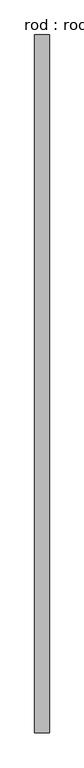
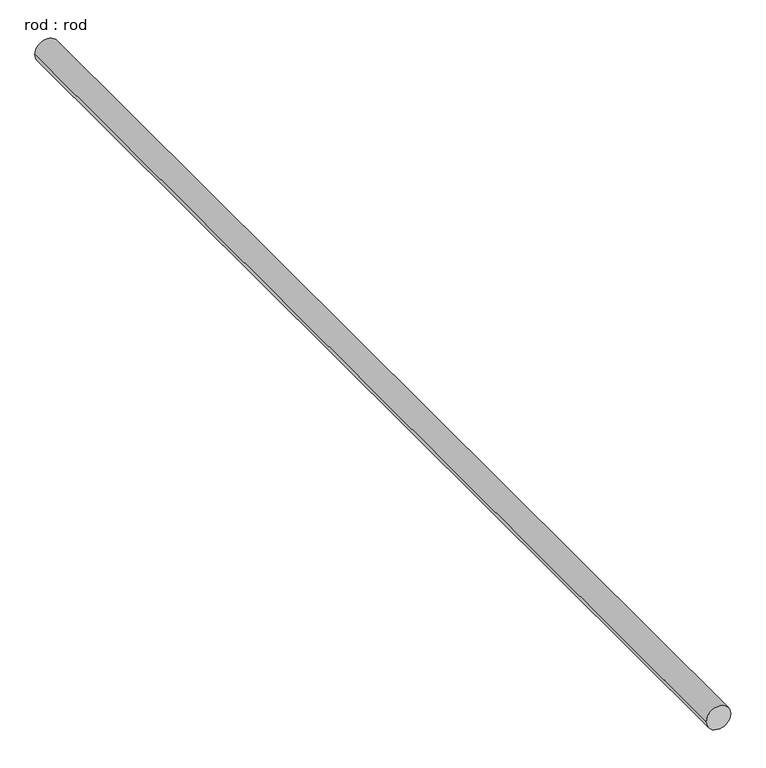
"""IFC4 building model written with IfcOpenShell, lengths in millimetres: proxy geometry, rod : rod."""

from ifc_helpers import new_model, si_unit, point, frame, frame_2d, origin, place, context, project, spatial, circle_curve, trimmed, segment, composite_curve, outline, extrude, source, transform, mapped, element, save


def rod_rod_24f0e566(model_context):
    return source(origin(), model_context, "Body", "SweptSolid", [
        extrude(outline(composite_curve([segment(trimmed(circle_curve(frame_2d((0.0108462, 0.0)), 200.0), [point((0.0108462, 200.0))], [point((0.0108462, -200.0))], False, "CARTESIAN"), True, "CONTINUOUS"), segment(trimmed(circle_curve(frame_2d((0.0108462, 0.0)), 200.0), [point((0.0108462, -200.0))], [point((0.0108462, 200.0))], False, "CARTESIAN"), True, "CONTINUOUS")], self_intersect=False)), frame((0.0, -5469.7713847, 0.0), z_axis=(0.0, 1.0, 0.0), x_axis=(0.0, 0.0, 1.0)), (0.0, 0.0, 1.0), 19125.0),
    ])


if __name__ == "__main__":
    model = new_model("IFC4")
    model_context = context("Model", 3, world=origin())
    ifc_project = project(units=[si_unit("LENGTHUNIT", "METRE", prefix="MILLI")], contexts=[model_context])
    site = spatial("IfcSite", under=ifc_project)
    building = spatial("IfcBuilding", under=site)
    placement = place(None, origin())
    rod_rod_shape = rod_rod_24f0e566(model_context)
    element("IfcBuildingElementProxy", 1, Name="rod : rod", ObjectType="rod : rod", at=placement, inside=building, context=model_context, shape_type="MappedRepresentation", body=[
        mapped(rod_rod_shape, transform((0.0, 0.0, 0.0), x_axis=(1.0, 0.0, 0.0), y_axis=(0.0, 1.0, 0.0), z_axis=(0.0, 0.0, 1.0))),
    ])
    save(model, "model.ifc")

# Revit data of these elements
# Type "rod : rod"
#   Default Elevation = 0
